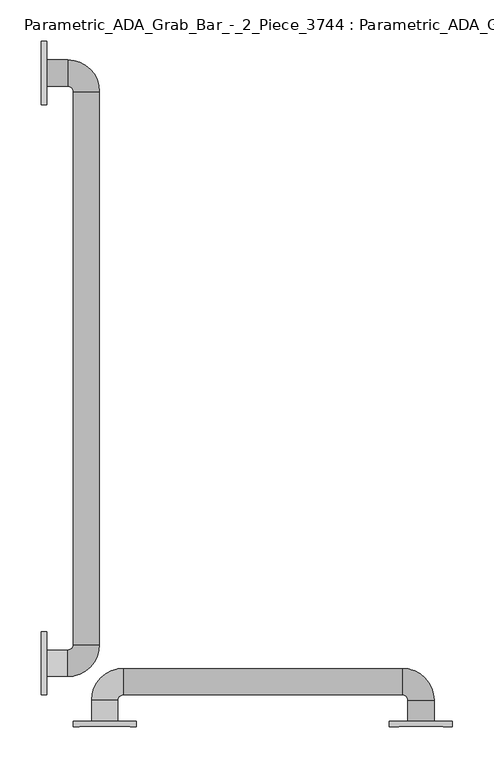
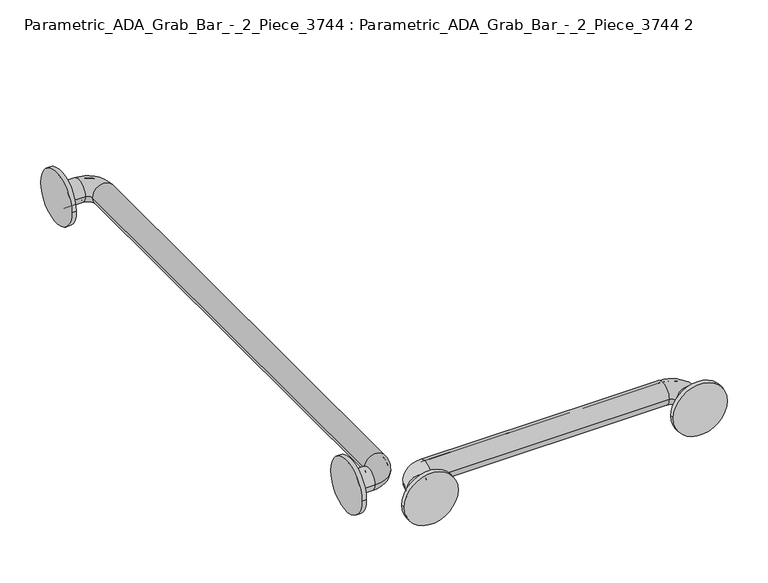
"""IFC4 building model written with IfcOpenShell, lengths in millimetres: proxy geometry, Parametric_ADA_Grab_Bar_-_2_Piece_3744 : Parametric_ADA_Grab_Bar_-_2_Piece_3744 2."""

import ifcopenshell
import ifcopenshell.guid

model = None  # the IFC model being written
_history = None  # IfcOwnerHistory: only IFC2X3 demands one
_inside = {}  # id of a spatial element -> (the spatial element, [elements in it])
_under = {}  # id of a project, library or spatial element -> (it, [spatial elements below it])
_declared = {}  # id of a project -> (the project, [libraries it declares])
_typed = {}  # id of a type object -> (the type object, [elements of that type])
_made_of = {}  # id of a material, layer set ... -> (it, [elements and type objects made of it])


def new_model(schema):
    """Start an empty IFC model of exactly this schema.

    Asked for "IFC4X3", IfcOpenShell would pick the latest addendum, in which some entities
    have other attributes; the version numbers below select the first issue.
    IFC2X3 requires an IfcOwnerHistory on every rooted entity: one is made here for all.
    """
    global model, _history
    if schema == "IFC4X3":
        model = ifcopenshell.file(schema_version=(4, 3, 0, 0))
    else:
        model = ifcopenshell.file(schema=schema)
    _inside.clear()
    _under.clear()
    _declared.clear()
    _typed.clear()
    _made_of.clear()
    _history = None
    if model.schema == "IFC2X3":
        org = make("IfcOrganization", Name="unknown")
        user = make(
            "IfcPersonAndOrganization",
            ThePerson=make("IfcPerson", FamilyName="unknown"),
            TheOrganization=org,
        )
        app = make(
            "IfcApplication",
            ApplicationDeveloper=org,
            Version="unknown",
            ApplicationFullName="unknown",
            ApplicationIdentifier="unknown",
        )
        _history = make(
            "IfcOwnerHistory",
            OwningUser=user,
            OwningApplication=app,
            ChangeAction="ADDED",
            CreationDate=0,
        )
    return model


def make(cls, **values):
    """One entity of the class cls with the attributes given. An attribute that is None is left unset."""
    return model.create_entity(
        cls, **{name: value for name, value in values.items() if value is not None}
    )


def rooted(cls, **values):
    """An entity with a GlobalId (a new one), such as an element, a storey or a relation."""
    return make(cls, GlobalId=ifcopenshell.guid.new(), OwnerHistory=_history, **values)


def si_unit(unit_type, name, prefix=None):
    """IfcSIUnit, for example si_unit("LENGTHUNIT", "METRE", prefix="MILLI")."""
    return make("IfcSIUnit", UnitType=unit_type, Prefix=prefix, Name=name)


def assignment(units):
    """IfcUnitAssignment: the units of a project."""
    return None if units is None else make("IfcUnitAssignment", Units=units)


def point(xyz):
    """IfcCartesianPoint."""
    return None if xyz is None else make("IfcCartesianPoint", Coordinates=xyz)


def direction(xyz):
    """IfcDirection."""
    return None if xyz is None else make("IfcDirection", DirectionRatios=xyz)


def frame(location, z_axis=None, x_axis=None):
    """IfcAxis2Placement3D, a coordinate frame: its origin and axes. An axis left out is left unset."""
    return make(
        "IfcAxis2Placement3D",
        Location=point(location),
        Axis=direction(z_axis),
        RefDirection=direction(x_axis),
    )


def frame_2d(location, x_axis=None):
    """IfcAxis2Placement2D, a coordinate frame in the plane: its origin and x axis."""
    return make(
        "IfcAxis2Placement2D", Location=point(location), RefDirection=direction(x_axis)
    )


def origin():
    """The frame at (0, 0, 0) with its axes left unset."""
    return frame((0.0, 0.0, 0.0))


def place(relative_to, where):
    """IfcLocalPlacement: puts the frame where relative to a parent placement (None: the world)."""
    return make(
        "IfcLocalPlacement", PlacementRelTo=relative_to, RelativePlacement=where
    )


def context(
    kind, dimensions, precision=None, world=None, true_north=None, identifier=None
):
    """IfcGeometricRepresentationContext, for example the 3D "Model" context."""
    return make(
        "IfcGeometricRepresentationContext",
        ContextIdentifier=identifier,
        ContextType=kind,
        CoordinateSpaceDimension=dimensions,
        Precision=precision,
        WorldCoordinateSystem=world,
        TrueNorth=true_north,
    )


def project(units=None, contexts=None):
    """IfcProject with its units and contexts."""
    return rooted(
        "IfcProject",
        Name="project",
        RepresentationContexts=contexts,
        UnitsInContext=assignment(units),
    )


def spatial(cls, under=None, at=None, **own):
    """A site, building, storey or space (cls), placed at a placement, below another one or the project."""
    s = rooted(cls, ObjectPlacement=at, **own)
    if under is not None:
        _under.setdefault(under.id(), (under, []))[1].append(s)
    return s


def polyline(points):
    """IfcPolyline through the points."""
    return make("IfcPolyline", Points=[point(p) for p in points])


def circle_curve(where, radius):
    """IfcCircle in the frame where."""
    return make("IfcCircle", Position=where, Radius=radius)


def ellipse_curve(where, semi_axis1, semi_axis2):
    """IfcEllipse in the frame where."""
    return make(
        "IfcEllipse", Position=where, SemiAxis1=semi_axis1, SemiAxis2=semi_axis2
    )


def trimmed(basis, trim1, trim2, sense, master):
    """IfcTrimmedCurve: the piece of a basis curve between two trims."""
    return make(
        "IfcTrimmedCurve",
        BasisCurve=basis,
        Trim1=trim1,
        Trim2=trim2,
        SenseAgreement=sense,
        MasterRepresentation=master,
    )


def segment(curve, same_sense, transition):
    """IfcCompositeCurveSegment."""
    return make(
        "IfcCompositeCurveSegment",
        Transition=transition,
        SameSense=same_sense,
        ParentCurve=curve,
    )


def composite_curve(segments, self_intersect=None):
    """IfcCompositeCurve: segments joined end to end."""
    return make("IfcCompositeCurve", Segments=segments, SelfIntersect=self_intersect)


def outline(outer, holes=None, kind="AREA"):
    """IfcArbitraryClosedProfileDef: a profile drawn as a closed curve; with holes, ...WithVoids."""
    if holes is None:
        return make("IfcArbitraryClosedProfileDef", ProfileType=kind, OuterCurve=outer)
    return make(
        "IfcArbitraryProfileDefWithVoids",
        ProfileType=kind,
        OuterCurve=outer,
        InnerCurves=holes,
    )


def extrude(swept, where, along, depth):
    """IfcExtrudedAreaSolid: the profile swept, set in the frame where, extruded along a direction by depth."""
    return make(
        "IfcExtrudedAreaSolid",
        SweptArea=swept,
        Position=where,
        ExtrudedDirection=direction(along),
        Depth=depth,
    )


def shape(context_of_items, identifier, shape_type, items):
    """IfcShapeRepresentation: the items that make up one representation, for example the "Body"."""
    return make(
        "IfcShapeRepresentation",
        ContextOfItems=context_of_items,
        RepresentationIdentifier=identifier,
        RepresentationType=shape_type,
        Items=items,
    )


def source(mapping_origin, context_of_items, identifier, shape_type, items):
    """IfcRepresentationMap: a shape defined once, which mapped items show again and again."""
    return make(
        "IfcRepresentationMap",
        MappingOrigin=mapping_origin,
        MappedRepresentation=shape(context_of_items, identifier, shape_type, items),
    )


def transform(
    local_origin,
    x_axis=None,
    y_axis=None,
    z_axis=None,
    scale=None,
    scale2=None,
    scale3=None,
    uniform=True,
):
    """IfcCartesianTransformationOperator3D, or its non-uniform kind. x_axis, y_axis, z_axis: its Axis1, 2, 3."""
    if uniform:
        return make(
            "IfcCartesianTransformationOperator3D",
            Axis1=direction(x_axis),
            Axis2=direction(y_axis),
            LocalOrigin=point(local_origin),
            Scale=scale,
            Axis3=direction(z_axis),
        )
    return make(
        "IfcCartesianTransformationOperator3DnonUniform",
        Axis1=direction(x_axis),
        Axis2=direction(y_axis),
        LocalOrigin=point(local_origin),
        Scale=scale,
        Axis3=direction(z_axis),
        Scale2=scale2,
        Scale3=scale3,
    )


def mapped(mapping_source, mapping_target):
    """IfcMappedItem: shows the shape of a source again, moved by a transform."""
    return make(
        "IfcMappedItem", MappingSource=mapping_source, MappingTarget=mapping_target
    )


def made_of(thing, what):
    """Note that an element or type object is made of a material, layer set ...; save() writes the relation."""
    if what is not None:
        _made_of.setdefault(what.id(), (what, []))[1].append(thing)
    return thing


def element(
    cls,
    number,
    at=None,
    inside=None,
    cuts=None,
    type_object=None,
    material=None,
    context=None,
    identifier="Body",
    shape_type=None,
    held_by="IfcProductDefinitionShape",
    body=None,
    shapes=None,
    **own,
):
    """One element of the class cls, such as IfcWall. Its Tag is "e" and its number.

    at: its placement. inside: the storey or other place that contains it. cuts: it is an
    opening in that element (IfcRelVoidsElement). A single representation is given by context,
    identifier, shape_type and body (its items); several are given by shapes. held_by: the class
    of the entity that holds the representations. save() writes the other relations.
    """
    e = rooted(cls, Tag="e%d" % number, ObjectPlacement=at, **own)
    if body is not None:
        shapes = [shape(context, identifier, shape_type, body)]
    if shapes is not None:
        e.Representation = make(held_by, Representations=shapes)
    if inside is not None:
        _inside.setdefault(inside.id(), (inside, []))[1].append(e)
    if cuts is not None:
        rooted(
            "IfcRelVoidsElement", RelatingBuildingElement=cuts, RelatedOpeningElement=e
        )
    if type_object is not None:
        _typed.setdefault(type_object.id(), (type_object, []))[1].append(e)
    return made_of(e, material)


def aggregate(whole, parts):
    """IfcRelAggregates: a whole, such as a stair, and the parts it consists of."""
    return rooted("IfcRelAggregates", RelatingObject=whole, RelatedObjects=parts)


def save(model, path):
    """Write the relations noted so far, then the file.

    IfcRelAggregates (storeys below a building ...), IfcRelContainedInSpatialStructure (elements
    in a storey), IfcRelDefinesByType, IfcRelAssociatesMaterial and IfcRelDeclares: one each for
    every whole, place, type object, material and project.
    """
    for whole, parts in _under.values():
        aggregate(whole, parts)
    for where, things in _inside.values():
        rooted(
            "IfcRelContainedInSpatialStructure",
            RelatedElements=things,
            RelatingStructure=where,
        )
    for kind, things in _typed.values():
        rooted("IfcRelDefinesByType", RelatedObjects=things, RelatingType=kind)
    for what, things in _made_of.values():
        rooted("IfcRelAssociatesMaterial", RelatedObjects=things, RelatingMaterial=what)
    for by, libraries in _declared.values():
        rooted("IfcRelDeclares", RelatingContext=by, RelatedDefinitions=libraries)
    model.write(path)


def plane_surface(at):
    """IfcPlane: the flat surface through the origin of the frame at, square to its z axis."""
    return make("IfcPlane", Position=at)


def cylinder_surface(at, radius):
    """IfcCylindricalSurface: all points at the distance radius from the z axis of the frame at."""
    return make("IfcCylindricalSurface", Position=at, Radius=radius)


def revolved_surface(curve, axis_point, axis_direction):
    """IfcSurfaceOfRevolution: the curve turned about the line through axis_point along axis_direction."""
    return make(
        "IfcSurfaceOfRevolution",
        SweptCurve=make("IfcArbitraryOpenProfileDef", ProfileType="CURVE", Curve=curve),
        AxisPosition=make("IfcAxis1Placement", Location=point(axis_point), Axis=direction(axis_direction)),
    )


def advanced_brep(points, edges, surfaces, faces):
    """IfcAdvancedBrep: a solid bounded by faces that lie on surfaces and meet in shared edges.

    An edge is (start, end): straight between two places in points (the first is 0);
    or (start, end, curve); or (start, end, curve, False) where it runs against its curve.
    A face is (place in surfaces, loops), or (place, loops, False) where it looks against
    its surface's normal. A loop lists edges by number (the first is 1), with a minus sign
    where the edge is run from its end to its start. The first loop is the outer one.
    """
    corners = [point(p) for p in points]
    vertices = [make("IfcVertexPoint", VertexGeometry=c) for c in corners]
    made = []
    for start, end, *more in edges:
        made.append(
            make(
                "IfcEdgeCurve",
                EdgeStart=vertices[start],
                EdgeEnd=vertices[end],
                EdgeGeometry=more[0] if more else make("IfcPolyline", Points=[corners[start], corners[end]]),
                SameSense=more[1] if len(more) > 1 else True,
            )
        )
    hull = []
    for where, loops, *sense in faces:
        bounds = []
        for j, loop in enumerate(loops):
            ring = [make("IfcOrientedEdge", EdgeElement=made[abs(k) - 1], Orientation=k > 0) for k in loop]
            bounds.append(
                make(
                    "IfcFaceOuterBound" if j == 0 else "IfcFaceBound",
                    Bound=make("IfcEdgeLoop", EdgeList=ring),
                    Orientation=True,
                )
            )
        hull.append(make("IfcAdvancedFace", Bounds=bounds, FaceSurface=surfaces[where], SameSense=sense[0] if sense else True))
    return make("IfcAdvancedBrep", Outer=make("IfcClosedShell", CfsFaces=hull))


def parametric_ada_grab_bar_2_piece_3744_parametric_ada_grab_bar_cda52879(model_context):
    return source(origin(), model_context, "Body", "SolidModel", [
        advanced_brep(
        [(6.35, 785.01875, 838.2), (6.35, 816.76875, 838.2), (6.35, 788.19375, 838.2), (6.35, 813.59375, 838.2), (31.75, 785.01875, 838.2), (31.75, 816.76875, 838.2), (31.75, 788.19375, 838.2), (31.75, 813.59375, 838.2), (69.85, 778.66875, 838.2), (38.1, 778.66875, 838.2), (66.675, 778.66875, 838.2), (41.275, 778.66875, 838.2), (38.1, 111.91875, 838.2), (69.85, 111.91875, 838.2), (41.275, 111.91875, 838.2), (66.675, 111.91875, 838.2), (31.75, 73.81875, 838.2), (31.75, 105.56875, 838.2), (31.75, 76.99375, 838.2), (31.75, 102.39375, 838.2), (6.35, 105.56875, 838.2), (6.35, 73.81875, 838.2), (6.35, 102.39375, 838.2), (6.35, 76.99375, 838.2)],
        [
            (0, 1, circle_curve(frame((6.35, 800.89375, 838.2), z_axis=(-1.0, 0.0, 0.0), x_axis=(0.0, 1.0, 0.0)), 15.875)),
            (1, 0, circle_curve(frame((6.35, 800.89375, 838.2), z_axis=(-1.0, 0.0, 0.0), x_axis=(0.0, 1.0, 0.0)), 15.875)),
            (2, 3, circle_curve(frame((6.35, 800.89375, 838.2), z_axis=(1.0, 0.0, 0.0), x_axis=(0.0, 1.0, 0.0)), 12.7)),
            (3, 2, circle_curve(frame((6.35, 800.89375, 838.2), z_axis=(1.0, 0.0, 0.0), x_axis=(0.0, 1.0, 0.0)), 12.7)),
            (0, 4),
            (4, 5, circle_curve(frame((31.75, 800.89375, 838.2), z_axis=(-1.0, 0.0, 0.0), x_axis=(0.0, 1.0, 0.0)), 15.875)),
            (5, 1),
            (5, 4, circle_curve(frame((31.75, 800.89375, 838.2), z_axis=(-1.0, 0.0, 0.0), x_axis=(0.0, 1.0, 0.0)), 15.875)),
            (2, 6),
            (6, 7, circle_curve(frame((31.75, 800.89375, 838.2), z_axis=(1.0, 0.0, 0.0), x_axis=(0.0, 1.0, 0.0)), 12.7)),
            (7, 3),
            (7, 6, circle_curve(frame((31.75, 800.89375, 838.2), z_axis=(1.0, 0.0, 0.0), x_axis=(0.0, 1.0, 0.0)), 12.7)),
            (8, 5, circle_curve(frame((31.75, 778.66875, 838.2), z_axis=(0.0, 0.0, 1.0), x_axis=(0.0, 1.0, 0.0)), 38.1)),
            (4, 9, circle_curve(frame((31.75, 778.66875, 838.2), z_axis=(0.0, 0.0, -1.0), x_axis=(0.0, 1.0, 0.0)), 6.35)),
            (9, 8, circle_curve(frame((53.975, 778.66875, 838.2), z_axis=(0.0, 1.0, 0.0), x_axis=(1.0, 0.0, 0.0)), 15.875)),
            (8, 9, circle_curve(frame((53.975, 778.66875, 838.2), z_axis=(0.0, 1.0, 0.0), x_axis=(1.0, 0.0, 0.0)), 15.875)),
            (10, 7, circle_curve(frame((31.75, 778.66875, 838.2), z_axis=(0.0, 0.0, 1.0), x_axis=(0.0, 1.0, 0.0)), 34.925)),
            (6, 11, circle_curve(frame((31.75, 778.66875, 838.2), z_axis=(0.0, 0.0, -1.0), x_axis=(0.0, 1.0, 0.0)), 9.525)),
            (11, 10, circle_curve(frame((53.975, 778.66875, 838.2), z_axis=(0.0, -1.0, 0.0), x_axis=(1.0, 0.0, 0.0)), 12.7)),
            (10, 11, circle_curve(frame((53.975, 778.66875, 838.2), z_axis=(0.0, -1.0, 0.0), x_axis=(1.0, 0.0, 0.0)), 12.7)),
            (9, 12),
            (12, 13, circle_curve(frame((53.975, 111.91875, 838.2), z_axis=(0.0, 1.0, 0.0), x_axis=(1.0, 0.0, 0.0)), 15.875)),
            (13, 8),
            (13, 12, circle_curve(frame((53.975, 111.91875, 838.2), z_axis=(0.0, 1.0, 0.0), x_axis=(1.0, 0.0, 0.0)), 15.875)),
            (11, 14),
            (14, 15, circle_curve(frame((53.975, 111.91875, 838.2), z_axis=(0.0, -1.0, 0.0), x_axis=(1.0, 0.0, 0.0)), 12.7)),
            (15, 10),
            (15, 14, circle_curve(frame((53.975, 111.91875, 838.2), z_axis=(0.0, -1.0, 0.0), x_axis=(1.0, 0.0, 0.0)), 12.7)),
            (16, 13, circle_curve(frame((31.75, 111.91875, 838.2), z_axis=(0.0, 0.0, 1.0), x_axis=(1.0, 0.0, 0.0)), 38.1)),
            (12, 17, circle_curve(frame((31.75, 111.91875, 838.2), z_axis=(0.0, 0.0, -1.0), x_axis=(1.0, 0.0, 0.0)), 6.35)),
            (17, 16, circle_curve(frame((31.75, 89.69375, 838.2), z_axis=(1.0, -1.076610172186615e-12, 0.0), x_axis=(-1.076610172186615e-12, -1.0, 0.0)), 15.875)),
            (16, 17, circle_curve(frame((31.75, 89.69375, 838.2), z_axis=(1.0, 0.0, 0.0), x_axis=(0.0, -1.0, 0.0)), 15.875)),
            (18, 15, circle_curve(frame((31.75, 111.91875, 838.2), z_axis=(0.0, 0.0, 1.0), x_axis=(1.0, 0.0, 0.0)), 34.925)),
            (14, 19, circle_curve(frame((31.75, 111.91875, 838.2), z_axis=(0.0, 0.0, -1.0), x_axis=(1.0, 0.0, 0.0)), 9.525)),
            (19, 18, circle_curve(frame((31.75, 89.69375, 838.2), z_axis=(-1.0, 0.0, 0.0), x_axis=(0.0, -1.0, 0.0)), 12.7)),
            (18, 19, circle_curve(frame((31.75, 89.69375, 838.2), z_axis=(-1.0, 0.0, 0.0), x_axis=(0.0, -1.0, 0.0)), 12.7)),
            (20, 21, circle_curve(frame((6.35, 89.69375, 838.2), z_axis=(-1.0, 0.0, 0.0), x_axis=(0.0, -1.0, 0.0)), 15.875)),
            (21, 20, circle_curve(frame((6.35, 89.69375, 838.2), z_axis=(-1.0, 0.0, 0.0), x_axis=(0.0, -1.0, 0.0)), 15.875)),
            (22, 23, circle_curve(frame((6.35, 89.69375, 838.2), z_axis=(1.0, 0.0, 0.0), x_axis=(0.0, -1.0, 0.0)), 12.7)),
            (23, 22, circle_curve(frame((6.35, 89.69375, 838.2), z_axis=(1.0, 0.0, 0.0), x_axis=(0.0, -1.0, 0.0)), 12.7)),
            (17, 20),
            (21, 16),
            (19, 22),
            (23, 18),
        ],
        [
            plane_surface(frame((6.35, 800.89375, 838.2), z_axis=(-1.0, 0.0, 0.0), x_axis=(0.0, 0.0, 1.0))),
            cylinder_surface(frame((6.35, 800.89375, 838.2), z_axis=(-1.0, 0.0, 0.0), x_axis=(0.0, 1.0, 0.0)), 15.875),
            revolved_surface(polyline([(31.75, 813.59375, 838.2), (6.35, 813.59375, 838.2)]), (6.35, 800.89375, 838.2), (1.0, 0.0, 0.0)),
            revolved_surface(trimmed(ellipse_curve(frame((31.75, 800.89375, 838.2), z_axis=(-1.0, 0.0, 0.0), x_axis=(0.0, 1.0, 0.0)), 15.875, 15.875), [point((31.75, 785.01875, 838.2))], [point((31.75, 816.76875, 838.2))], True, "CARTESIAN"), (31.75, 778.66875, 838.2), (0.0, 0.0, -1.0)),
            revolved_surface(trimmed(ellipse_curve(frame((31.75, 800.89375, 838.2), z_axis=(-1.0, 0.0, 0.0), x_axis=(0.0, 1.0, 0.0)), 15.875, 15.875), [point((31.75, 816.76875, 838.2))], [point((31.75, 785.01875, 838.2))], True, "CARTESIAN"), (31.75, 778.66875, 838.2), (0.0, 0.0, -1.0)),
            revolved_surface(trimmed(ellipse_curve(frame((31.75, 800.89375, 838.2), z_axis=(1.0, 0.0, 0.0), x_axis=(0.0, 1.0, 0.0)), 12.7, 12.7), [point((31.75, 788.19375, 838.2))], [point((31.75, 813.59375, 838.2))], True, "CARTESIAN"), (31.75, 778.66875, 838.2), (0.0, 0.0, -1.0)),
            revolved_surface(trimmed(ellipse_curve(frame((31.75, 800.89375, 838.2), z_axis=(1.0, 0.0, 0.0), x_axis=(0.0, 1.0, 0.0)), 12.7, 12.7), [point((31.75, 813.59375, 838.2))], [point((31.75, 788.19375, 838.2))], True, "CARTESIAN"), (31.75, 778.66875, 838.2), (0.0, 0.0, -1.0)),
            cylinder_surface(frame((53.975, 778.66875, 838.2), z_axis=(0.0, 1.0, 0.0), x_axis=(1.0, 0.0, 0.0)), 15.875),
            revolved_surface(polyline([(66.675, 111.91875000000005, 838.2), (66.675, 778.66875, 838.2)]), (53.975, 778.66875, 838.2), (0.0, -1.0, 0.0)),
            revolved_surface(trimmed(ellipse_curve(frame((53.975, 111.91875, 838.2), z_axis=(0.0, 1.0, 0.0), x_axis=(1.0, 0.0, 0.0)), 15.875, 15.875), [point((38.1, 111.91875, 838.2))], [point((69.85, 111.91875, 838.2))], True, "CARTESIAN"), (31.75, 111.91875, 838.2), (0.0, 0.0, -1.0)),
            revolved_surface(trimmed(ellipse_curve(frame((53.975, 111.91875, 838.2), z_axis=(0.0, 1.0, 0.0), x_axis=(1.0, 0.0, 0.0)), 15.875, 15.875), [point((69.85, 111.91875, 838.2))], [point((38.1, 111.91875, 838.2))], True, "CARTESIAN"), (31.75, 111.91875, 838.2), (0.0, 0.0, -1.0)),
            revolved_surface(trimmed(ellipse_curve(frame((53.975, 111.91875, 838.2), z_axis=(0.0, -1.0, 0.0), x_axis=(1.0, 0.0, 0.0)), 12.7, 12.7), [point((41.275, 111.91875, 838.2))], [point((66.675, 111.91875, 838.2))], True, "CARTESIAN"), (31.75, 111.91875, 838.2), (0.0, 0.0, -1.0)),
            revolved_surface(trimmed(ellipse_curve(frame((53.975, 111.91875, 838.2), z_axis=(0.0, -1.0, 0.0), x_axis=(1.0, 0.0, 0.0)), 12.7, 12.7), [point((66.675, 111.91875, 838.2))], [point((41.275, 111.91875, 838.2))], True, "CARTESIAN"), (31.75, 111.91875, 838.2), (0.0, 0.0, -1.0)),
            plane_surface(frame((6.35, 89.69375, 838.2), z_axis=(-1.0, 0.0, 0.0), x_axis=(0.0, 0.0, 1.0))),
            cylinder_surface(frame((31.75, 89.69375, 838.2), z_axis=(1.0, 0.0, 0.0), x_axis=(0.0, -1.0, 0.0)), 15.875),
            revolved_surface(polyline([(6.350000000000001, 76.99374999999999, 838.2), (31.75, 76.99374999999999, 838.2)]), (31.75, 89.69375, 838.2), (-1.0, 0.0, 0.0)),
        ],
        [
            (0, [[1, 2], [3, 4]]),
            (1, [[-1, 5, 6, 7]]),
            (1, [[-2, -7, 8, -5]]),
            (2, [[-3, 9, 10, 11]]),
            (2, [[-4, -11, 12, -9]]),
            (3, [[13, -6, 14, 15]]),
            (4, [[-14, -8, -13, 16]]),
            (5, [[17, -10, 18, 19]]),
            (6, [[-18, -12, -17, 20]]),
            (7, [[-15, 21, 22, 23]]),
            (7, [[-16, -23, 24, -21]]),
            (8, [[-19, 25, 26, 27]]),
            (8, [[-20, -27, 28, -25]]),
            (9, [[29, -22, 30, 31]]),
            (10, [[-30, -24, -29, 32]]),
            (11, [[33, -26, 34, 35]]),
            (12, [[-34, -28, -33, 36]]),
            (13, [[37, 38], [39, 40]]),
            (14, [[-31, 41, -38, 42]]),
            (14, [[-32, -42, -37, -41]]),
            (15, [[-35, 43, -40, 44]]),
            (15, [[-36, -44, -39, -43]]),
        ],
    ),
        advanced_brep(
        [(92.075, 19.84375, 838.2), (60.325, 19.84375, 838.2), (88.9, 19.84375, 838.2), (63.5, 19.84375, 838.2), (92.075, 45.24375, 838.2), (60.325, 45.24375, 838.2), (88.9, 45.24375, 838.2), (63.5, 45.24375, 838.2), (98.425, 83.34375, 838.2), (98.425, 51.59375, 838.2), (98.425, 80.16875, 838.2), (98.425, 54.76875, 838.2), (434.975, 51.59375, 838.2), (434.975, 83.34375, 838.2), (434.975, 54.76875, 838.2), (434.975, 80.16875, 838.2), (473.075, 45.24375, 838.2), (441.325, 45.24375, 838.2), (469.9, 45.24375, 838.2), (444.5, 45.24375, 838.2), (441.325, 19.84375, 838.2), (473.075, 19.84375, 838.2), (444.5, 19.84375, 838.2), (469.9, 19.84375, 838.2)],
        [
            (0, 1, circle_curve(frame((76.2, 19.84375, 838.2), z_axis=(0.0, -1.0, 0.0), x_axis=(-1.0, 0.0, 0.0)), 15.875)),
            (1, 0, circle_curve(frame((76.2, 19.84375, 838.2), z_axis=(0.0, -1.0, 0.0), x_axis=(-1.0, 0.0, 0.0)), 15.875)),
            (2, 3, circle_curve(frame((76.2, 19.84375, 838.2), z_axis=(0.0, 1.0, 0.0), x_axis=(-1.0, 0.0, 0.0)), 12.7)),
            (3, 2, circle_curve(frame((76.2, 19.84375, 838.2), z_axis=(0.0, 1.0, 0.0), x_axis=(-1.0, 0.0, 0.0)), 12.7)),
            (0, 4),
            (4, 5, circle_curve(frame((76.2, 45.24375, 838.2), z_axis=(0.0, -1.0, 0.0), x_axis=(-1.0, 0.0, 0.0)), 15.875)),
            (5, 1),
            (5, 4, circle_curve(frame((76.2, 45.24375, 838.2), z_axis=(0.0, -1.0, 0.0), x_axis=(-1.0, 0.0, 0.0)), 15.875)),
            (2, 6),
            (6, 7, circle_curve(frame((76.2, 45.24375, 838.2), z_axis=(0.0, 1.0, 0.0), x_axis=(-1.0, 0.0, 0.0)), 12.7)),
            (7, 3),
            (7, 6, circle_curve(frame((76.2, 45.24375, 838.2), z_axis=(0.0, 1.0, 0.0), x_axis=(-1.0, 0.0, 0.0)), 12.7)),
            (8, 5, circle_curve(frame((98.425, 45.24375, 838.2), z_axis=(0.0, 0.0, 1.0), x_axis=(-1.0, 0.0, 0.0)), 38.1)),
            (4, 9, circle_curve(frame((98.425, 45.24375, 838.2), z_axis=(0.0, 0.0, -1.0), x_axis=(-1.0, 0.0, 0.0)), 6.35)),
            (9, 8, circle_curve(frame((98.425, 67.46875, 838.2), z_axis=(-1.0, 0.0, 0.0), x_axis=(0.0, 1.0, 0.0)), 15.875)),
            (8, 9, circle_curve(frame((98.425, 67.46875, 838.2), z_axis=(-1.0, 0.0, 0.0), x_axis=(0.0, 1.0, 0.0)), 15.875)),
            (10, 7, circle_curve(frame((98.425, 45.24375, 838.2), z_axis=(0.0, 0.0, 1.0), x_axis=(-1.0, 0.0, 0.0)), 34.925)),
            (6, 11, circle_curve(frame((98.425, 45.24375, 838.2), z_axis=(0.0, 0.0, -1.0), x_axis=(-1.0, 0.0, 0.0)), 9.525)),
            (11, 10, circle_curve(frame((98.425, 67.46875, 838.2), z_axis=(1.0, 0.0, 0.0), x_axis=(0.0, 1.0, 0.0)), 12.7)),
            (10, 11, circle_curve(frame((98.425, 67.46875, 838.2), z_axis=(1.0, 0.0, 0.0), x_axis=(0.0, 1.0, 0.0)), 12.7)),
            (9, 12),
            (12, 13, circle_curve(frame((434.975, 67.46875, 838.2), z_axis=(-1.0, 0.0, 0.0), x_axis=(0.0, 1.0, 0.0)), 15.875)),
            (13, 8),
            (13, 12, circle_curve(frame((434.975, 67.46875, 838.2), z_axis=(-1.0, 0.0, 0.0), x_axis=(0.0, 1.0, 0.0)), 15.875)),
            (11, 14),
            (14, 15, circle_curve(frame((434.975, 67.46875, 838.2), z_axis=(1.0, 0.0, 0.0), x_axis=(0.0, 1.0, 0.0)), 12.7)),
            (15, 10),
            (15, 14, circle_curve(frame((434.975, 67.46875, 838.2), z_axis=(1.0, 0.0, 0.0), x_axis=(0.0, 1.0, 0.0)), 12.7)),
            (16, 13, circle_curve(frame((434.975, 45.24375, 838.2), z_axis=(0.0, 0.0, 1.0), x_axis=(0.0, 1.0, 0.0)), 38.1)),
            (12, 17, circle_curve(frame((434.975, 45.24375, 838.2), z_axis=(0.0, 0.0, -1.0), x_axis=(0.0, 1.0, 0.0)), 6.35)),
            (17, 16, circle_curve(frame((457.2, 45.24375, 838.2), z_axis=(1.0730574585078145e-12, 1.0, 0.0), x_axis=(1.0, -1.0730574585078145e-12, 0.0)), 15.875)),
            (16, 17, circle_curve(frame((457.2, 45.24375, 838.2), z_axis=(0.0, 1.0, 0.0), x_axis=(1.0, 0.0, 0.0)), 15.875)),
            (18, 15, circle_curve(frame((434.975, 45.24375, 838.2), z_axis=(0.0, 0.0, 1.0), x_axis=(0.0, 1.0, 0.0)), 34.925)),
            (14, 19, circle_curve(frame((434.975, 45.24375, 838.2), z_axis=(0.0, 0.0, -1.0), x_axis=(0.0, 1.0, 0.0)), 9.525)),
            (19, 18, circle_curve(frame((457.2, 45.24375, 838.2), z_axis=(0.0, -1.0, 0.0), x_axis=(1.0, 0.0, 0.0)), 12.7)),
            (18, 19, circle_curve(frame((457.2, 45.24375, 838.2), z_axis=(0.0, -1.0, 0.0), x_axis=(1.0, 0.0, 0.0)), 12.7)),
            (20, 21, circle_curve(frame((457.2, 19.84375, 838.2), z_axis=(0.0, -1.0, 0.0), x_axis=(1.0, 0.0, 0.0)), 15.875)),
            (21, 20, circle_curve(frame((457.2, 19.84375, 838.2), z_axis=(0.0, -1.0, 0.0), x_axis=(1.0, 0.0, 0.0)), 15.875)),
            (22, 23, circle_curve(frame((457.2, 19.84375, 838.2), z_axis=(0.0, 1.0, 0.0), x_axis=(1.0, 0.0, 0.0)), 12.7)),
            (23, 22, circle_curve(frame((457.2, 19.84375, 838.2), z_axis=(0.0, 1.0, 0.0), x_axis=(1.0, 0.0, 0.0)), 12.7)),
            (17, 20),
            (21, 16),
            (19, 22),
            (23, 18),
        ],
        [
            plane_surface(frame((76.2, 19.84375, 838.2), z_axis=(0.0, -1.0, 0.0), x_axis=(0.0, 0.0, 1.0))),
            cylinder_surface(frame((76.2, 19.84375, 838.2), z_axis=(0.0, -1.0, 0.0), x_axis=(-1.0, 0.0, 0.0)), 15.875),
            revolved_surface(polyline([(63.5, 45.24375, 838.2), (63.5, 19.84375, 838.2)]), (76.2, 19.84375, 838.2), (0.0, 1.0, 0.0)),
            revolved_surface(trimmed(ellipse_curve(frame((76.2, 45.24375, 838.2), z_axis=(0.0, -1.0, 0.0), x_axis=(-1.0, 0.0, 0.0)), 15.875, 15.875), [point((92.075, 45.24375, 838.2))], [point((60.325, 45.24375, 838.2))], True, "CARTESIAN"), (98.425, 45.24375, 838.2), (0.0, 0.0, -1.0)),
            revolved_surface(trimmed(ellipse_curve(frame((76.2, 45.24375, 838.2), z_axis=(0.0, -1.0, 0.0), x_axis=(-1.0, 0.0, 0.0)), 15.875, 15.875), [point((60.325, 45.24375, 838.2))], [point((92.075, 45.24375, 838.2))], True, "CARTESIAN"), (98.425, 45.24375, 838.2), (0.0, 0.0, -1.0)),
            revolved_surface(trimmed(ellipse_curve(frame((76.2, 45.24375, 838.2), z_axis=(0.0, 1.0, 0.0), x_axis=(-1.0, 0.0, 0.0)), 12.7, 12.7), [point((88.9, 45.24375, 838.2))], [point((63.5, 45.24375, 838.2))], True, "CARTESIAN"), (98.425, 45.24375, 838.2), (0.0, 0.0, -1.0)),
            revolved_surface(trimmed(ellipse_curve(frame((76.2, 45.24375, 838.2), z_axis=(0.0, 1.0, 0.0), x_axis=(-1.0, 0.0, 0.0)), 12.7, 12.7), [point((63.5, 45.24375, 838.2))], [point((88.9, 45.24375, 838.2))], True, "CARTESIAN"), (98.425, 45.24375, 838.2), (0.0, 0.0, -1.0)),
            cylinder_surface(frame((98.425, 67.46875, 838.2), z_axis=(-1.0, 0.0, 0.0), x_axis=(0.0, 1.0, 0.0)), 15.875),
            revolved_surface(polyline([(434.975, 80.16875, 838.2), (98.425, 80.16875, 838.2)]), (98.425, 67.46875, 838.2), (1.0, 0.0, 0.0)),
            revolved_surface(trimmed(ellipse_curve(frame((434.975, 67.46875, 838.2), z_axis=(-1.0, 0.0, 0.0), x_axis=(0.0, 1.0, 0.0)), 15.875, 15.875), [point((434.975, 51.59375, 838.2))], [point((434.975, 83.34375, 838.2))], True, "CARTESIAN"), (434.975, 45.24375, 838.2), (0.0, 0.0, -1.0)),
            revolved_surface(trimmed(ellipse_curve(frame((434.975, 67.46875, 838.2), z_axis=(-1.0, 0.0, 0.0), x_axis=(0.0, 1.0, 0.0)), 15.875, 15.875), [point((434.975, 83.34375, 838.2))], [point((434.975, 51.59375, 838.2))], True, "CARTESIAN"), (434.975, 45.24375, 838.2), (0.0, 0.0, -1.0)),
            revolved_surface(trimmed(ellipse_curve(frame((434.975, 67.46875, 838.2), z_axis=(1.0, 0.0, 0.0), x_axis=(0.0, 1.0, 0.0)), 12.7, 12.7), [point((434.975, 54.76875, 838.2))], [point((434.975, 80.16875, 838.2))], True, "CARTESIAN"), (434.975, 45.24375, 838.2), (0.0, 0.0, -1.0)),
            revolved_surface(trimmed(ellipse_curve(frame((434.975, 67.46875, 838.2), z_axis=(1.0, 0.0, 0.0), x_axis=(0.0, 1.0, 0.0)), 12.7, 12.7), [point((434.975, 80.16875, 838.2))], [point((434.975, 54.76875, 838.2))], True, "CARTESIAN"), (434.975, 45.24375, 838.2), (0.0, 0.0, -1.0)),
            plane_surface(frame((457.2, 19.84375, 838.2), z_axis=(0.0, -1.0, 0.0), x_axis=(0.0, 0.0, 1.0))),
            cylinder_surface(frame((457.2, 45.24375, 838.2), z_axis=(0.0, 1.0, 0.0), x_axis=(1.0, 0.0, 0.0)), 15.875),
            revolved_surface(polyline([(469.9, 19.84375, 838.2), (469.9, 45.24375, 838.2)]), (457.2, 45.24375, 838.2), (0.0, -1.0, 0.0)),
        ],
        [
            (0, [[1, 2], [3, 4]]),
            (1, [[-1, 5, 6, 7]]),
            (1, [[-2, -7, 8, -5]]),
            (2, [[-3, 9, 10, 11]]),
            (2, [[-4, -11, 12, -9]]),
            (3, [[13, -6, 14, 15]]),
            (4, [[-14, -8, -13, 16]]),
            (5, [[17, -10, 18, 19]]),
            (6, [[-18, -12, -17, 20]]),
            (7, [[-15, 21, 22, 23]]),
            (7, [[-16, -23, 24, -21]]),
            (8, [[-19, 25, 26, 27]]),
            (8, [[-20, -27, 28, -25]]),
            (9, [[29, -22, 30, 31]]),
            (10, [[-30, -24, -29, 32]]),
            (11, [[33, -26, 34, 35]]),
            (12, [[-34, -28, -33, 36]]),
            (13, [[37, 38], [39, 40]]),
            (14, [[-31, 41, -38, 42]]),
            (14, [[-32, -42, -37, -41]]),
            (15, [[-35, 43, -40, 44]]),
            (15, [[-36, -44, -39, -43]]),
        ],
    ),
        extrude(outline(composite_curve([segment(trimmed(circle_curve(frame_2d((89.69375, 838.2)), 38.1), [point((51.59375, 838.2))], [point((127.79375, 838.2))], False, "CARTESIAN"), True, "CONTINUOUS"), segment(trimmed(circle_curve(frame_2d((89.69375, 838.2)), 38.1), [point((127.79375, 838.2))], [point((51.59375, 838.2))], False, "CARTESIAN"), True, "CONTINUOUS")], self_intersect=False)), frame((0.0, 0.0, 0.0), z_axis=(1.0, 0.0, 0.0), x_axis=(0.0, 1.0, 0.0)), (0.0, 0.0, 1.0), 6.35),
        extrude(outline(composite_curve([segment(trimmed(circle_curve(frame_2d((800.89375, 838.2)), 38.1), [point((762.79375, 838.2))], [point((838.99375, 838.2))], False, "CARTESIAN"), True, "CONTINUOUS"), segment(trimmed(circle_curve(frame_2d((800.89375, 838.2)), 38.1), [point((838.99375, 838.2))], [point((762.79375, 838.2))], False, "CARTESIAN"), True, "CONTINUOUS")], self_intersect=False)), frame((0.0, 0.0, 0.0), z_axis=(1.0, 0.0, 0.0), x_axis=(0.0, 1.0, 0.0)), (0.0, 0.0, 1.0), 6.35),
        extrude(outline(composite_curve([segment(trimmed(circle_curve(frame_2d((838.2, 457.2)), 38.1), [point((838.2, 419.1))], [point((838.2, 495.3))], False, "CARTESIAN"), True, "CONTINUOUS"), segment(trimmed(circle_curve(frame_2d((838.2, 457.2)), 38.1), [point((838.2, 495.3))], [point((838.2, 419.1))], False, "CARTESIAN"), True, "CONTINUOUS")], self_intersect=False)), frame((0.0, 13.49375, 0.0), z_axis=(0.0, 1.0, 0.0), x_axis=(0.0, 0.0, 1.0)), (0.0, 0.0, 1.0), 6.35),
        extrude(outline(composite_curve([segment(trimmed(circle_curve(frame_2d((838.2, 76.2)), 38.1), [point((838.2, 38.1))], [point((838.2, 114.3))], False, "CARTESIAN"), True, "CONTINUOUS"), segment(trimmed(circle_curve(frame_2d((838.2, 76.2)), 38.1), [point((838.2, 114.3))], [point((838.2, 38.1))], False, "CARTESIAN"), True, "CONTINUOUS")], self_intersect=False)), frame((0.0, 13.49375, 0.0), z_axis=(0.0, 1.0, 0.0), x_axis=(0.0, 0.0, 1.0)), (0.0, 0.0, 1.0), 6.35),
    ])


if __name__ == "__main__":
    model = new_model("IFC4")
    model_context = context("Model", 3, world=origin())
    ifc_project = project(units=[si_unit("LENGTHUNIT", "METRE", prefix="MILLI")], contexts=[model_context])
    site = spatial("IfcSite", under=ifc_project)
    building = spatial("IfcBuilding", under=site)
    placement = place(None, origin())
    parametric_ada_grab_bar_2_piece_3744_parametric_ada_grab_bar_shape = parametric_ada_grab_bar_2_piece_3744_parametric_ada_grab_bar_cda52879(model_context)
    element("IfcBuildingElementProxy", 1, Name="Parametric_ADA_Grab_Bar_-_2_Piece_3744 : Parametric_ADA_Grab_Bar_-_2_Piece_3744 2", ObjectType="Parametric_ADA_Grab_Bar_-_2_Piece_3744 : Parametric_ADA_Grab_Bar_-_2_Piece_3744 2", at=placement, inside=building, context=model_context, shape_type="MappedRepresentation", body=[
        mapped(parametric_ada_grab_bar_2_piece_3744_parametric_ada_grab_bar_shape, transform((0.0, 0.0, 0.0), x_axis=(1.0, 0.0, 0.0), y_axis=(0.0, 1.0, 0.0), z_axis=(0.0, 0.0, 1.0))),
    ])
    save(model, "model.ifc")

# Revit data of these elements
# Type "Parametric_ADA_Grab_Bar_-_2_Piece_3744 : Parametric_ADA_Grab_Bar_-_2_Piece_3744 2"
#   Keynote = "M10281313.01"
#   Grab bar length (42" min) = 2' - 4"
#   Grab bar height = 2' - 9"
#   Grab bar Length (36" min) = 1' - 3"
#   Face of Wall to Grab bar (6" max) = 0' - 3"
#   Face of Wall to Grab bar (12" max) = 0' - 3"
# Element 1 (IfcBuildingElementProxy, "Parametric_ADA_Grab_Bar_-_2_Piece_3744 : Parametric_ADA_Grab_Bar_-_2_Piece_3744 2")
#   Materials on its faces: "Stainless Steel"
# Materials
#   "Stainless Steel": class "Metal", colour RGB 0 0 0, transparency 0, Description = "Stainless Steel 18/8", Cost = 0
